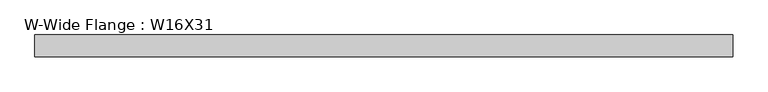
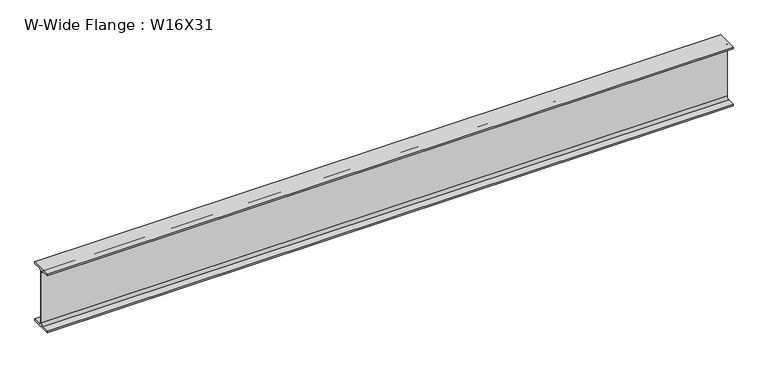
"""IFC4 building model written with IfcOpenShell, lengths in millimetres: beam geometry, W-Wide Flange : W16X31."""

from ifc_helpers import new_model, si_unit, point, frame, frame_2d, origin, place, context, project, spatial, polyline, circle_curve, trimmed, segment, composite_curve, outline, extrude, source, transform, mapped, element, save


def w_wide_flange_w16x31_9accb003(model_context):
    return source(origin(), model_context, "Body", "SweptSolid", [
        extrude(outline(composite_curve([segment(polyline([(70.231, -190.754), (70.231, -201.93), (-70.231, -201.93), (-70.231, -190.754), (-20.8915, -190.754)]), True, "CONTINUOUS"), segment(trimmed(circle_curve(frame_2d((-20.8915, -173.355)), 17.399), [point((-20.8915, -190.754))], [point((-3.4925, -173.355))], True, "CARTESIAN"), True, "CONTINUOUS"), segment(polyline([(-3.4925, -173.355), (-3.4925, 173.355)]), True, "CONTINUOUS"), segment(trimmed(circle_curve(frame_2d((-20.8915, 173.355)), 17.399), [point((-3.4925, 173.355))], [point((-20.8915, 190.754))], True, "CARTESIAN"), True, "CONTINUOUS"), segment(polyline([(-20.8915, 190.754), (-70.231, 190.754), (-70.231, 201.93), (70.231, 201.93), (70.231, 190.754), (20.8915, 190.754)]), True, "CONTINUOUS"), segment(trimmed(circle_curve(frame_2d((20.8915, 173.355)), 17.399), [point((20.8915, 190.754))], [point((3.4925, 173.355))], True, "CARTESIAN"), True, "CONTINUOUS"), segment(polyline([(3.4925, 173.355), (3.4925, -173.355)]), True, "CONTINUOUS"), segment(trimmed(circle_curve(frame_2d((20.8915, -173.355)), 17.399), [point((3.4925, -173.355))], [point((20.8915, -190.754))], True, "CARTESIAN"), True, "CONTINUOUS"), segment(polyline([(20.8915, -190.754), (70.231, -190.754)]), True, "CONTINUOUS")], self_intersect=False)), frame((-2235.2, 0.0, 0.0), z_axis=(1.0, 0.0, 0.0), x_axis=(0.0, 1.0, 0.0)), (0.0, 0.0, 1.0), 4470.4),
    ])


if __name__ == "__main__":
    model = new_model("IFC4")
    model_context = context("Model", 3, world=origin())
    ifc_project = project(units=[si_unit("LENGTHUNIT", "METRE", prefix="MILLI")], contexts=[model_context])
    site = spatial("IfcSite", under=ifc_project)
    building = spatial("IfcBuilding", under=site)
    placement = place(None, origin())
    w_wide_flange_w16x31_shape = w_wide_flange_w16x31_9accb003(model_context)
    element("IfcBeam", 1, ObjectType="W-Wide Flange : W16X31", at=placement, inside=building, context=model_context, shape_type="MappedRepresentation", body=[
        mapped(w_wide_flange_w16x31_shape, transform((0.0, 0.0, 0.0), x_axis=(1.0, 0.0, 0.0), y_axis=(0.0, 1.0, 0.0), z_axis=(0.0, 0.0, 1.0))),
    ])
    save(model, "model.ifc")

# Revit data of these elements
# Type "W-Wide Flange : W16X31"
#   Assembly Code = "B10"
#   W = 31
#   Length [instance default] = 5' - 0"
#   bf = 0' - 5.53"
#   d = 1' - 3.9"
#   k = 0' - 1 1/8"
#   k2 = 0' - 0.685"
#   tf = 0' - 0.44"
#   tw = 0' - 0.275"
#   A = 0.0634028 SF
#   Structural Material [instance default] = Steel ASTM A992
# Element 1 (IfcBeam, "W-Wide Flange : W16X31")
#   Materials on its faces: "Steel ASTM A992"
# Materials
#   "Steel ASTM A992": class "Metal", colour RGB 199 199 199, transparency 0, Description = "Structural steel 50ksi", Cost = 0
